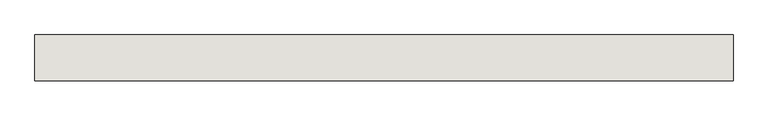
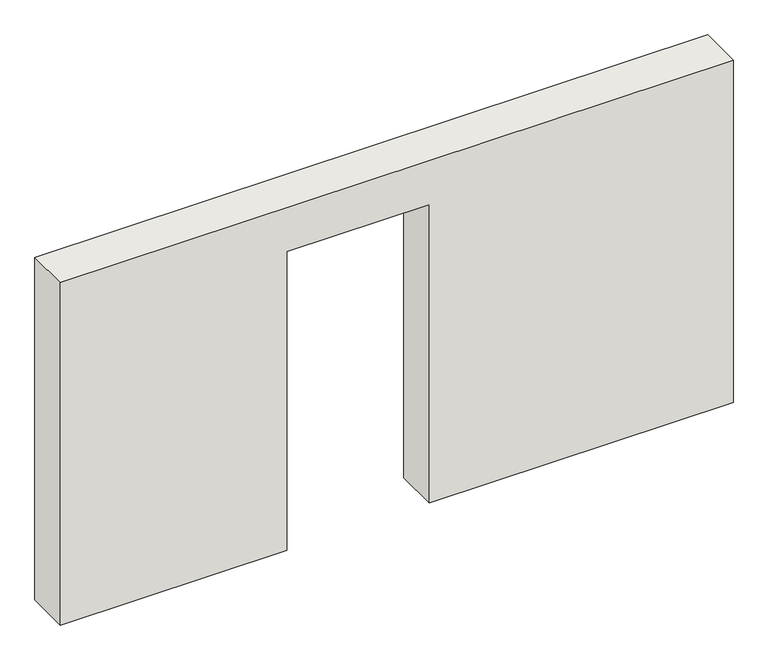
"""IFC4 building model written with IfcOpenShell, lengths in millimetres: wall geometry, 0_3d."""

from ifc_helpers import new_model, si_unit, frame, origin, place, context, project, spatial, polyline, outline, extrude, source, transform, mapped, element, save


def wall_d88cb43b(model_context):
    return source(origin(), model_context, "Body", "SweptSolid", [
        extrude(outline(polyline([(2510.0, 2935.0), (0.0, 2935.0), (0.0, 5350.0), (2880.0, 5350.0), (2880.0, 0.0), (0.0, 0.0), (0.0, 1800.0), (2510.0, 1800.0), (2510.0, 2935.0)])), frame((0.0, 0.0, 0.0), z_axis=(0.0, 1.0, 0.0), x_axis=(0.0, 0.0, 1.0)), (0.0, 0.0, 1.0), 350.0),
    ])


if __name__ == "__main__":
    model = new_model("IFC4")
    model_context = context("Model", 3, world=origin())
    ifc_project = project(units=[si_unit("LENGTHUNIT", "METRE", prefix="MILLI")], contexts=[model_context])
    site = spatial("IfcSite", under=ifc_project)
    building = spatial("IfcBuilding", under=site)
    placement = place(None, origin())
    wall_shape = wall_d88cb43b(model_context)
    element("IfcWall", 1, ObjectType="0_3d", at=placement, inside=building, context=model_context, shape_type="MappedRepresentation", body=[
        mapped(wall_shape, transform((0.0, 0.0, 0.0), x_axis=(1.0, 0.0, 0.0), y_axis=(0.0, 1.0, 0.0), z_axis=(0.0, 0.0, 1.0))),
    ])
    save(model, "model.ifc")

# Revit data of these elements
# Element 1 (IfcWall, "0_3d")
#   Materials on its faces: "holzschalung"
# Materials
#   "holzschalung": class "Unassigned", colour RGB 128 128 128, transparency 0
